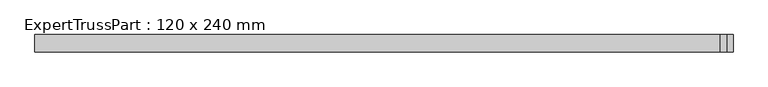
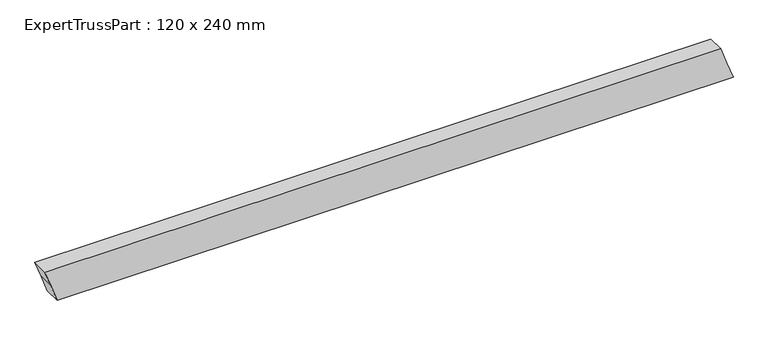
"""IFC4 building model written with IfcOpenShell, lengths in millimetres: beam geometry, ExpertTrussPart : 120 x 240 mm."""

import ifcopenshell
import ifcopenshell.guid

model = None  # the IFC model being written
_history = None  # IfcOwnerHistory: only IFC2X3 demands one
_inside = {}  # id of a spatial element -> (the spatial element, [elements in it])
_under = {}  # id of a project, library or spatial element -> (it, [spatial elements below it])
_declared = {}  # id of a project -> (the project, [libraries it declares])
_typed = {}  # id of a type object -> (the type object, [elements of that type])
_made_of = {}  # id of a material, layer set ... -> (it, [elements and type objects made of it])


def new_model(schema):
    """Start an empty IFC model of exactly this schema.

    Asked for "IFC4X3", IfcOpenShell would pick the latest addendum, in which some entities
    have other attributes; the version numbers below select the first issue.
    IFC2X3 requires an IfcOwnerHistory on every rooted entity: one is made here for all.
    """
    global model, _history
    if schema == "IFC4X3":
        model = ifcopenshell.file(schema_version=(4, 3, 0, 0))
    else:
        model = ifcopenshell.file(schema=schema)
    _inside.clear()
    _under.clear()
    _declared.clear()
    _typed.clear()
    _made_of.clear()
    _history = None
    if model.schema == "IFC2X3":
        org = make("IfcOrganization", Name="unknown")
        user = make(
            "IfcPersonAndOrganization",
            ThePerson=make("IfcPerson", FamilyName="unknown"),
            TheOrganization=org,
        )
        app = make(
            "IfcApplication",
            ApplicationDeveloper=org,
            Version="unknown",
            ApplicationFullName="unknown",
            ApplicationIdentifier="unknown",
        )
        _history = make(
            "IfcOwnerHistory",
            OwningUser=user,
            OwningApplication=app,
            ChangeAction="ADDED",
            CreationDate=0,
        )
    return model


def make(cls, **values):
    """One entity of the class cls with the attributes given. An attribute that is None is left unset."""
    return model.create_entity(
        cls, **{name: value for name, value in values.items() if value is not None}
    )


def rooted(cls, **values):
    """An entity with a GlobalId (a new one), such as an element, a storey or a relation."""
    return make(cls, GlobalId=ifcopenshell.guid.new(), OwnerHistory=_history, **values)


def si_unit(unit_type, name, prefix=None):
    """IfcSIUnit, for example si_unit("LENGTHUNIT", "METRE", prefix="MILLI")."""
    return make("IfcSIUnit", UnitType=unit_type, Prefix=prefix, Name=name)


def assignment(units):
    """IfcUnitAssignment: the units of a project."""
    return None if units is None else make("IfcUnitAssignment", Units=units)


def point(xyz):
    """IfcCartesianPoint."""
    return None if xyz is None else make("IfcCartesianPoint", Coordinates=xyz)


def direction(xyz):
    """IfcDirection."""
    return None if xyz is None else make("IfcDirection", DirectionRatios=xyz)


def frame(location, z_axis=None, x_axis=None):
    """IfcAxis2Placement3D, a coordinate frame: its origin and axes. An axis left out is left unset."""
    return make(
        "IfcAxis2Placement3D",
        Location=point(location),
        Axis=direction(z_axis),
        RefDirection=direction(x_axis),
    )


def origin():
    """The frame at (0, 0, 0) with its axes left unset."""
    return frame((0.0, 0.0, 0.0))


def place(relative_to, where):
    """IfcLocalPlacement: puts the frame where relative to a parent placement (None: the world)."""
    return make(
        "IfcLocalPlacement", PlacementRelTo=relative_to, RelativePlacement=where
    )


def context(
    kind, dimensions, precision=None, world=None, true_north=None, identifier=None
):
    """IfcGeometricRepresentationContext, for example the 3D "Model" context."""
    return make(
        "IfcGeometricRepresentationContext",
        ContextIdentifier=identifier,
        ContextType=kind,
        CoordinateSpaceDimension=dimensions,
        Precision=precision,
        WorldCoordinateSystem=world,
        TrueNorth=true_north,
    )


def project(units=None, contexts=None):
    """IfcProject with its units and contexts."""
    return rooted(
        "IfcProject",
        Name="project",
        RepresentationContexts=contexts,
        UnitsInContext=assignment(units),
    )


def spatial(cls, under=None, at=None, **own):
    """A site, building, storey or space (cls), placed at a placement, below another one or the project."""
    s = rooted(cls, ObjectPlacement=at, **own)
    if under is not None:
        _under.setdefault(under.id(), (under, []))[1].append(s)
    return s


def polyline(points):
    """IfcPolyline through the points."""
    return make("IfcPolyline", Points=[point(p) for p in points])


def outline(outer, holes=None, kind="AREA"):
    """IfcArbitraryClosedProfileDef: a profile drawn as a closed curve; with holes, ...WithVoids."""
    if holes is None:
        return make("IfcArbitraryClosedProfileDef", ProfileType=kind, OuterCurve=outer)
    return make(
        "IfcArbitraryProfileDefWithVoids",
        ProfileType=kind,
        OuterCurve=outer,
        InnerCurves=holes,
    )


def extrude(swept, where, along, depth):
    """IfcExtrudedAreaSolid: the profile swept, set in the frame where, extruded along a direction by depth."""
    return make(
        "IfcExtrudedAreaSolid",
        SweptArea=swept,
        Position=where,
        ExtrudedDirection=direction(along),
        Depth=depth,
    )


def shape(context_of_items, identifier, shape_type, items):
    """IfcShapeRepresentation: the items that make up one representation, for example the "Body"."""
    return make(
        "IfcShapeRepresentation",
        ContextOfItems=context_of_items,
        RepresentationIdentifier=identifier,
        RepresentationType=shape_type,
        Items=items,
    )


def source(mapping_origin, context_of_items, identifier, shape_type, items):
    """IfcRepresentationMap: a shape defined once, which mapped items show again and again."""
    return make(
        "IfcRepresentationMap",
        MappingOrigin=mapping_origin,
        MappedRepresentation=shape(context_of_items, identifier, shape_type, items),
    )


def transform(
    local_origin,
    x_axis=None,
    y_axis=None,
    z_axis=None,
    scale=None,
    scale2=None,
    scale3=None,
    uniform=True,
):
    """IfcCartesianTransformationOperator3D, or its non-uniform kind. x_axis, y_axis, z_axis: its Axis1, 2, 3."""
    if uniform:
        return make(
            "IfcCartesianTransformationOperator3D",
            Axis1=direction(x_axis),
            Axis2=direction(y_axis),
            LocalOrigin=point(local_origin),
            Scale=scale,
            Axis3=direction(z_axis),
        )
    return make(
        "IfcCartesianTransformationOperator3DnonUniform",
        Axis1=direction(x_axis),
        Axis2=direction(y_axis),
        LocalOrigin=point(local_origin),
        Scale=scale,
        Axis3=direction(z_axis),
        Scale2=scale2,
        Scale3=scale3,
    )


def mapped(mapping_source, mapping_target):
    """IfcMappedItem: shows the shape of a source again, moved by a transform."""
    return make(
        "IfcMappedItem", MappingSource=mapping_source, MappingTarget=mapping_target
    )


def made_of(thing, what):
    """Note that an element or type object is made of a material, layer set ...; save() writes the relation."""
    if what is not None:
        _made_of.setdefault(what.id(), (what, []))[1].append(thing)
    return thing


def element(
    cls,
    number,
    at=None,
    inside=None,
    cuts=None,
    type_object=None,
    material=None,
    context=None,
    identifier="Body",
    shape_type=None,
    held_by="IfcProductDefinitionShape",
    body=None,
    shapes=None,
    **own,
):
    """One element of the class cls, such as IfcWall. Its Tag is "e" and its number.

    at: its placement. inside: the storey or other place that contains it. cuts: it is an
    opening in that element (IfcRelVoidsElement). A single representation is given by context,
    identifier, shape_type and body (its items); several are given by shapes. held_by: the class
    of the entity that holds the representations. save() writes the other relations.
    """
    e = rooted(cls, Tag="e%d" % number, ObjectPlacement=at, **own)
    if body is not None:
        shapes = [shape(context, identifier, shape_type, body)]
    if shapes is not None:
        e.Representation = make(held_by, Representations=shapes)
    if inside is not None:
        _inside.setdefault(inside.id(), (inside, []))[1].append(e)
    if cuts is not None:
        rooted(
            "IfcRelVoidsElement", RelatingBuildingElement=cuts, RelatedOpeningElement=e
        )
    if type_object is not None:
        _typed.setdefault(type_object.id(), (type_object, []))[1].append(e)
    return made_of(e, material)


def aggregate(whole, parts):
    """IfcRelAggregates: a whole, such as a stair, and the parts it consists of."""
    return rooted("IfcRelAggregates", RelatingObject=whole, RelatedObjects=parts)


def save(model, path):
    """Write the relations noted so far, then the file.

    IfcRelAggregates (storeys below a building ...), IfcRelContainedInSpatialStructure (elements
    in a storey), IfcRelDefinesByType, IfcRelAssociatesMaterial and IfcRelDeclares: one each for
    every whole, place, type object, material and project.
    """
    for whole, parts in _under.values():
        aggregate(whole, parts)
    for where, things in _inside.values():
        rooted(
            "IfcRelContainedInSpatialStructure",
            RelatedElements=things,
            RelatingStructure=where,
        )
    for kind, things in _typed.values():
        rooted("IfcRelDefinesByType", RelatedObjects=things, RelatingType=kind)
    for what, things in _made_of.values():
        rooted("IfcRelAssociatesMaterial", RelatedObjects=things, RelatingMaterial=what)
    for by, libraries in _declared.values():
        rooted("IfcRelDeclares", RelatingContext=by, RelatedDefinitions=libraries)
    model.write(path)


def experttrusspart_120_x_240_mm_cafd0cc5(model_context):
    return source(origin(), model_context, "Body", "SweptSolid", [
        extrude(outline(polyline([(240.0, -2408.8115274), (120.0, -2365.1350993), (0.0, -2321.4586712), (0.0, 2408.8115274), (120.0, 2365.1350993), (240.0, 2321.4586712), (240.0, -2408.8115274)])), frame((0.0, -60.0, 0.0), z_axis=(0.0, 1.0, 0.0), x_axis=(0.0, 0.0, 1.0)), (0.0, 0.0, 1.0), 120.0),
    ])


if __name__ == "__main__":
    model = new_model("IFC4")
    model_context = context("Model", 3, world=origin())
    ifc_project = project(units=[si_unit("LENGTHUNIT", "METRE", prefix="MILLI")], contexts=[model_context])
    site = spatial("IfcSite", under=ifc_project)
    building = spatial("IfcBuilding", under=site)
    placement = place(None, origin())
    experttrusspart_120_x_240_mm_shape = experttrusspart_120_x_240_mm_cafd0cc5(model_context)
    element("IfcBeam", 1, ObjectType="ExpertTrussPart : 120 x 240 mm", at=placement, inside=building, context=model_context, shape_type="MappedRepresentation", body=[
        mapped(experttrusspart_120_x_240_mm_shape, transform((0.0, 0.0, 0.0), x_axis=(1.0, 0.0, 0.0), y_axis=(0.0, 1.0, 0.0), z_axis=(0.0, 0.0, 1.0))),
    ])
    save(model, "model.ifc")

# Revit data of these elements
# Type "ExpertTrussPart : 120 x 240 mm"
#   Expert Truss Part Name [instance default] = ""
#   _RT [instance default] = 100.00°
#   _RB [instance default] = 100.00°
#   _OR [instance default] = 10 mm
#   _OL [instance default] = 0 mm
#   _LT [instance default] = 100.00°
#   _LB [instance default] = 100.00°
#   _IR [instance default] = 0 mm
#   _IL [instance default] = 10 mm
#   _HR [instance default] = 110 mm
#   _HL [instance default] = 110 mm
#   Width = 120 mm
#   WF [instance default] = 60 mm
#   WB [instance default] = 60 mm
#   VR [instance default] = 10 mm
#   VL [instance default] = -10 mm
#   RT [instance default] = 10.00°
#   RB [instance default] = 10.00°
#   Piękny Parametr [instance default] = 180 mm
#   Height/2 [instance default] = 120 mm
#   Length [instance default] = 3000 mm
#   LT [instance default] = 10.00°
#   LB [instance default] = 10.00°
#   Height = 240 mm
#   HT [instance default] = 60 mm
#   HR [instance default] = 10 mm
#   HL [instance default] = 10 mm
#   HB [instance default] = 180 mm
#   Expert Truss Id [instance default] = 0
#   Material = Wood Standard
# Element 1 (IfcBeam, "ExpertTrussPart : 120 x 240 mm")
#   _RT = 110.00°
#   _RB = 70.00°
#   _OR = 0 mm
#   _LT = 70.00°
#   _LB = 110.00°
#   _IL = 0 mm
#   _HR = 120 mm
#   _HL = 120 mm
#   VR = 0 mm
#   VL = 0 mm
#   RT = 20.00°
#   RB = -20.00°
#   Piękny Parametr = 240 mm
#   LT = -20.00°
#   LB = 20.00°
#   HT = 120 mm
#   HR = 0 mm
#   HL = 0 mm
#   HB = 120 mm
#   Materials on its faces: "Wood Standard"
# Materials
#   "Wood Standard": class "Drewno", colour RGB 196 146 67, transparency 0, Cost = 0
